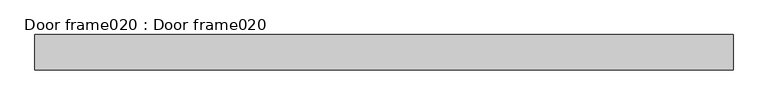
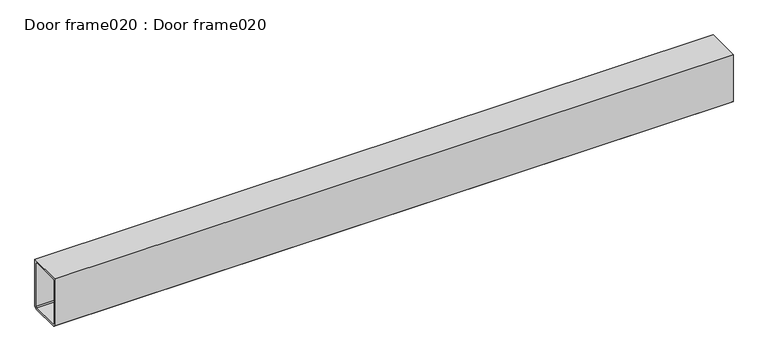
"""IFC4 building model written with IfcOpenShell, lengths in millimetres: proxy geometry, Door frame020 : Door frame020."""

from ifc_helpers import new_model, si_unit, frame, origin, place, context, project, spatial, polyline, outline, extrude, source, transform, mapped, element, save


def door_frame020_door_frame020_938791e3(model_context):
    return source(origin(), model_context, "Body", "SweptSolid", [
        extrude(outline(polyline([(9648.8015375, 37902.896), (9750.4015375, 37902.896), (9750.4015375, 37756.846), (9744.0515375, 37750.496), (9655.1515375, 37750.496), (9648.8015375, 37756.846), (9648.8015375, 37902.896)]), holes=[polyline([(9744.0515375, 37759.4762561), (9744.0515375, 37893.9157439), (9741.4212814, 37896.546), (9657.7817936, 37896.546), (9655.1515375, 37893.9157439), (9655.1515375, 37759.4762561), (9657.7817936, 37756.846), (9741.4212814, 37756.846), (9744.0515375, 37759.4762561)])]), frame((-9232.0719278, 0.0, 0.0), z_axis=(1.0, 0.0, 0.0), x_axis=(0.0, 1.0, 0.0)), (0.0, 0.0, 1.0), 1999.85),
    ])


if __name__ == "__main__":
    model = new_model("IFC4")
    model_context = context("Model", 3, world=origin())
    ifc_project = project(units=[si_unit("LENGTHUNIT", "METRE", prefix="MILLI")], contexts=[model_context])
    site = spatial("IfcSite", under=ifc_project)
    building = spatial("IfcBuilding", under=site)
    placement = place(None, origin())
    door_frame020_door_frame020_shape = door_frame020_door_frame020_938791e3(model_context)
    element("IfcBuildingElementProxy", 1, Name="Door frame020 : Door frame020", ObjectType="Door frame020 : Door frame020", at=placement, inside=building, context=model_context, shape_type="MappedRepresentation", body=[
        mapped(door_frame020_door_frame020_shape, transform((0.0, 0.0, 0.0), x_axis=(1.0, 0.0, 0.0), y_axis=(0.0, 1.0, 0.0), z_axis=(0.0, 0.0, 1.0))),
    ])
    save(model, "model.ifc")

# Revit data of these elements
# Type "Door frame020 : Door frame020"
#   NameOverride = "Door frame020"
# Element 1 (IfcBuildingElementProxy, "Door frame020 : Door frame020")
#   Materials on its faces: "DOOR FRAME: TUBE STEEL PROFILE - METALIZED, PRIMED & PAINTED (COLOR PER ARCHITECT)"
# Materials
#   "DOOR FRAME: TUBE STEEL PROFILE - METALIZED, PRIMED & PAINTED (COLOR PER ARCHITECT)": class "Unassigned", colour RGB 128 128 128, transparency 0, Cost = 0
